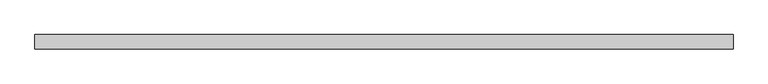
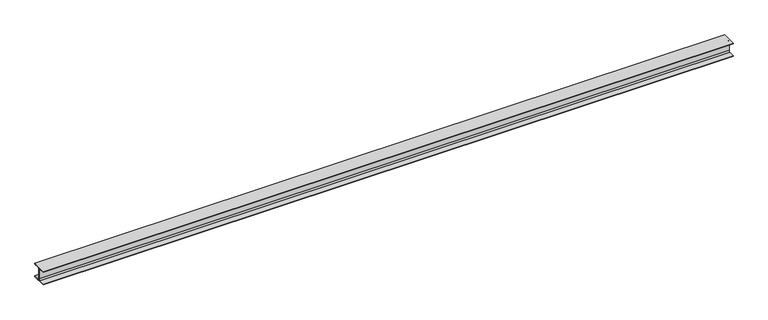
"""IFC4 building model written with IfcOpenShell, lengths in millimetres: beam geometry, NLRS_28_SF_LIB_stalen ligger HEB-AV-CWV-MMBS-SRP_gen_rsf : stalen ligger_gen__HEB 260."""

from ifc_helpers import new_model, si_unit, point, frame, frame_2d, origin, place, context, project, spatial, polyline, circle_curve, trimmed, segment, composite_curve, outline, extrude, source, transform, mapped, element, save


def beam_f33d2ea4(model_context):
    return source(origin(), model_context, "Body", "SweptSolid", [
        extrude(outline(composite_curve([segment(polyline([(-130.0, 112.5), (-130.0, 130.0), (130.0, 130.0), (130.0, 112.5), (29.0, 112.5)]), True, "CONTINUOUS"), segment(trimmed(circle_curve(frame_2d((29.0, 88.5)), 24.0), [point((29.0, 112.5))], [point((5.0, 88.5))], True, "CARTESIAN"), True, "CONTINUOUS"), segment(polyline([(5.0, 88.5), (5.0, -88.5)]), True, "CONTINUOUS"), segment(trimmed(circle_curve(frame_2d((29.0, -88.5)), 24.0), [point((5.0, -88.5))], [point((29.0, -112.5))], True, "CARTESIAN"), True, "CONTINUOUS"), segment(polyline([(29.0, -112.5), (130.0, -112.5), (130.0, -130.0), (-130.0, -130.0), (-130.0, -112.5), (-29.0, -112.5)]), True, "CONTINUOUS"), segment(trimmed(circle_curve(frame_2d((-29.0, -88.5)), 24.0), [point((-29.0, -112.5))], [point((-5.0, -88.5))], True, "CARTESIAN"), True, "CONTINUOUS"), segment(polyline([(-5.0, -88.5), (-5.0, 88.5)]), True, "CONTINUOUS"), segment(trimmed(circle_curve(frame_2d((-29.0, 88.5)), 24.0), [point((-5.0, 88.5))], [point((-29.0, 112.5))], True, "CARTESIAN"), True, "CONTINUOUS"), segment(polyline([(-29.0, 112.5), (-130.0, 112.5)]), True, "CONTINUOUS")], self_intersect=False)), frame((-6318.75, 0.0, 0.0), z_axis=(1.0, 0.0, 0.0), x_axis=(0.0, 1.0, 0.0)), (0.0, 0.0, 1.0), 12637.5),
    ])


if __name__ == "__main__":
    model = new_model("IFC4")
    model_context = context("Model", 3, world=origin())
    ifc_project = project(units=[si_unit("LENGTHUNIT", "METRE", prefix="MILLI")], contexts=[model_context])
    site = spatial("IfcSite", under=ifc_project)
    building = spatial("IfcBuilding", under=site)
    placement = place(None, origin())
    beam_shape = beam_f33d2ea4(model_context)
    element("IfcBeam", 1, ObjectType="NLRS_28_SF_LIB_stalen ligger HEB-AV-CWV-MMBS-SRP_gen_rsf : stalen ligger_gen__HEB 260", at=placement, inside=building, context=model_context, shape_type="MappedRepresentation", body=[
        mapped(beam_shape, transform((0.0, 0.0, 0.0), x_axis=(1.0, 0.0, 0.0), y_axis=(0.0, 1.0, 0.0), z_axis=(0.0, 0.0, 1.0))),
    ])
    save(model, "model.ifc")

# Revit data of these elements
# Type "NLRS_28_SF_LIB_stalen ligger HEB-AV-CWV-MMBS-SRP_gen_rsf : stalen ligger_gen__HEB 260"
#   Type IfcGUID = "0zo1UjqZ91lRsfCKsOOa5a"
#   IfcExportAs = "IfcBeamType"
#   Type Comments = "HEB260"
#   Model = " "
#   Manufacturer = " "
#   Fire Rating = " "
#   Description = "stalen ligger HEB260"
#   Assembly Code = "28.11"
#   ra = 24 mm
#   vz = 130 mm
#   vy = 130 mm
#   vpz = 130 mm
#   vpy = 130 mm
#   NLRS_C_lengte [instance default] = 1500 mm
#   Length [instance default] = 1500 mm
#   bf = 260 mm
#   d = 260 mm
#   tf = 17.5 mm
#   tw = 10 mm
#   Structural Material = NLRS_h2_staal_gen_rsf
#   Keynote = ""
# Element 1 (IfcBeam, "NLRS_28_SF_LIB_stalen ligger HEB-AV-CWV-MMBS-SRP_gen_rsf : stalen ligger_gen__HEB 260")
#   NLRS_C_lengte = 12637.5 mm
#   Materials on its faces: "NLRS_h2_staal_gen_rsf"
# Materials
#   "NLRS_h2_staal_gen_rsf": class "H - Metaal", colour RGB 189 187 185, transparency 0, Keynote = "h2", Manufacturer = "Revit Standards Foundation", URL = "www.revitstandards.org", Description = "staal", Cost = 0
